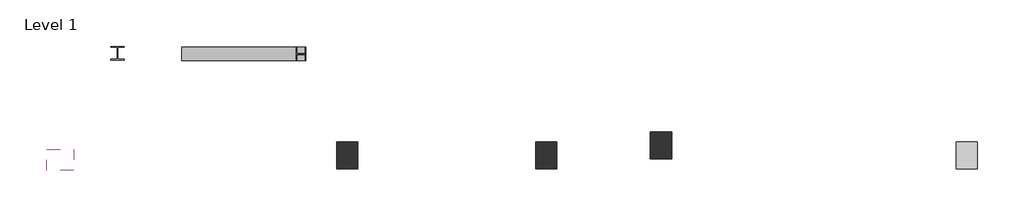
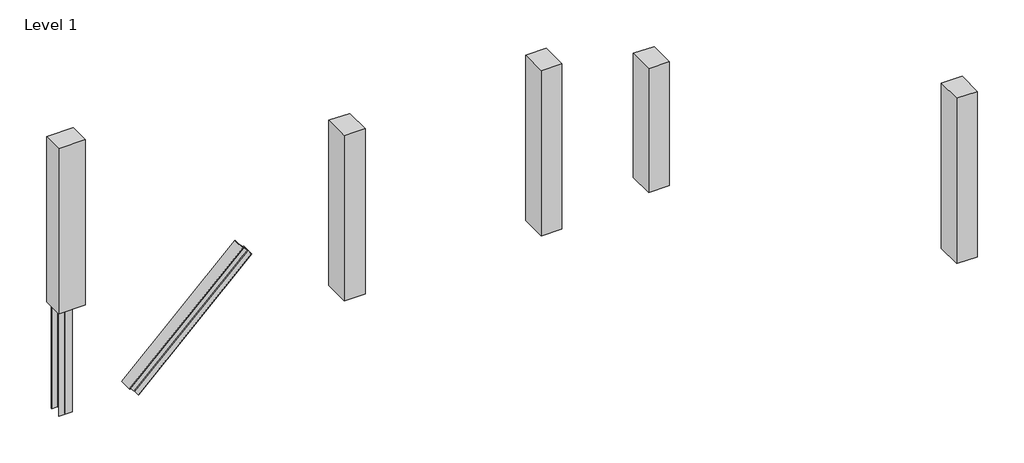
# One storey: 7 columns.
"""IFC4 building model written with IfcOpenShell, lengths in millimetres."""

import ifcopenshell
import ifcopenshell.guid

model = None  # the IFC model being written
_history = None  # IfcOwnerHistory: only IFC2X3 demands one
_inside = {}  # id of a spatial element -> (the spatial element, [elements in it])
_under = {}  # id of a project, library or spatial element -> (it, [spatial elements below it])
_declared = {}  # id of a project -> (the project, [libraries it declares])
_typed = {}  # id of a type object -> (the type object, [elements of that type])
_made_of = {}  # id of a material, layer set ... -> (it, [elements and type objects made of it])


def new_model(schema):
    """Start an empty IFC model of exactly this schema.

    Asked for "IFC4X3", IfcOpenShell would pick the latest addendum, in which some entities
    have other attributes; the version numbers below select the first issue.
    IFC2X3 requires an IfcOwnerHistory on every rooted entity: one is made here for all.
    """
    global model, _history
    if schema == "IFC4X3":
        model = ifcopenshell.file(schema_version=(4, 3, 0, 0))
    else:
        model = ifcopenshell.file(schema=schema)
    _inside.clear()
    _under.clear()
    _declared.clear()
    _typed.clear()
    _made_of.clear()
    _history = None
    if model.schema == "IFC2X3":
        org = make("IfcOrganization", Name="unknown")
        user = make(
            "IfcPersonAndOrganization",
            ThePerson=make("IfcPerson", FamilyName="unknown"),
            TheOrganization=org,
        )
        app = make(
            "IfcApplication",
            ApplicationDeveloper=org,
            Version="unknown",
            ApplicationFullName="unknown",
            ApplicationIdentifier="unknown",
        )
        _history = make(
            "IfcOwnerHistory",
            OwningUser=user,
            OwningApplication=app,
            ChangeAction="ADDED",
            CreationDate=0,
        )
    return model


def make(cls, **values):
    """One entity of the class cls with the attributes given. An attribute that is None is left unset."""
    return model.create_entity(
        cls, **{name: value for name, value in values.items() if value is not None}
    )


def rooted(cls, **values):
    """An entity with a GlobalId (a new one), such as an element, a storey or a relation."""
    return make(cls, GlobalId=ifcopenshell.guid.new(), OwnerHistory=_history, **values)


def si_unit(unit_type, name, prefix=None):
    """IfcSIUnit, for example si_unit("LENGTHUNIT", "METRE", prefix="MILLI")."""
    return make("IfcSIUnit", UnitType=unit_type, Prefix=prefix, Name=name)


def assignment(units):
    """IfcUnitAssignment: the units of a project."""
    return None if units is None else make("IfcUnitAssignment", Units=units)


def point(xyz):
    """IfcCartesianPoint."""
    return None if xyz is None else make("IfcCartesianPoint", Coordinates=xyz)


def direction(xyz):
    """IfcDirection."""
    return None if xyz is None else make("IfcDirection", DirectionRatios=xyz)


def frame(location, z_axis=None, x_axis=None):
    """IfcAxis2Placement3D, a coordinate frame: its origin and axes. An axis left out is left unset."""
    return make(
        "IfcAxis2Placement3D",
        Location=point(location),
        Axis=direction(z_axis),
        RefDirection=direction(x_axis),
    )


def frame_2d(location, x_axis=None):
    """IfcAxis2Placement2D, a coordinate frame in the plane: its origin and x axis."""
    return make(
        "IfcAxis2Placement2D", Location=point(location), RefDirection=direction(x_axis)
    )


def origin():
    """The frame at (0, 0, 0) with its axes left unset."""
    return frame((0.0, 0.0, 0.0))


def origin_with_axes():
    """The frame at (0, 0, 0) with the z axis (0, 0, 1) and the x axis (1, 0, 0) written out."""
    return frame((0.0, 0.0, 0.0), z_axis=(0.0, 0.0, 1.0), x_axis=(1.0, 0.0, 0.0))


def place(relative_to, where):
    """IfcLocalPlacement: puts the frame where relative to a parent placement (None: the world)."""
    return make(
        "IfcLocalPlacement", PlacementRelTo=relative_to, RelativePlacement=where
    )


def context(
    kind, dimensions, precision=None, world=None, true_north=None, identifier=None
):
    """IfcGeometricRepresentationContext, for example the 3D "Model" context."""
    return make(
        "IfcGeometricRepresentationContext",
        ContextIdentifier=identifier,
        ContextType=kind,
        CoordinateSpaceDimension=dimensions,
        Precision=precision,
        WorldCoordinateSystem=world,
        TrueNorth=true_north,
    )


def project(units=None, contexts=None):
    """IfcProject with its units and contexts."""
    return rooted(
        "IfcProject",
        Name="project",
        RepresentationContexts=contexts,
        UnitsInContext=assignment(units),
    )


def spatial(cls, under=None, at=None, **own):
    """A site, building, storey or space (cls), placed at a placement, below another one or the project."""
    s = rooted(cls, ObjectPlacement=at, **own)
    if under is not None:
        _under.setdefault(under.id(), (under, []))[1].append(s)
    return s


def polyline(points):
    """IfcPolyline through the points."""
    return make("IfcPolyline", Points=[point(p) for p in points])


def circle_curve(where, radius):
    """IfcCircle in the frame where."""
    return make("IfcCircle", Position=where, Radius=radius)


def trimmed(basis, trim1, trim2, sense, master):
    """IfcTrimmedCurve: the piece of a basis curve between two trims."""
    return make(
        "IfcTrimmedCurve",
        BasisCurve=basis,
        Trim1=trim1,
        Trim2=trim2,
        SenseAgreement=sense,
        MasterRepresentation=master,
    )


def segment(curve, same_sense, transition):
    """IfcCompositeCurveSegment."""
    return make(
        "IfcCompositeCurveSegment",
        Transition=transition,
        SameSense=same_sense,
        ParentCurve=curve,
    )


def composite_curve(segments, self_intersect=None):
    """IfcCompositeCurve: segments joined end to end."""
    return make("IfcCompositeCurve", Segments=segments, SelfIntersect=self_intersect)


def outline(outer, holes=None, kind="AREA"):
    """IfcArbitraryClosedProfileDef: a profile drawn as a closed curve; with holes, ...WithVoids."""
    if holes is None:
        return make("IfcArbitraryClosedProfileDef", ProfileType=kind, OuterCurve=outer)
    return make(
        "IfcArbitraryProfileDefWithVoids",
        ProfileType=kind,
        OuterCurve=outer,
        InnerCurves=holes,
    )


def extrude(swept, where, along, depth):
    """IfcExtrudedAreaSolid: the profile swept, set in the frame where, extruded along a direction by depth."""
    return make(
        "IfcExtrudedAreaSolid",
        SweptArea=swept,
        Position=where,
        ExtrudedDirection=direction(along),
        Depth=depth,
    )


def shape(context_of_items, identifier, shape_type, items):
    """IfcShapeRepresentation: the items that make up one representation, for example the "Body"."""
    return make(
        "IfcShapeRepresentation",
        ContextOfItems=context_of_items,
        RepresentationIdentifier=identifier,
        RepresentationType=shape_type,
        Items=items,
    )


def source(mapping_origin, context_of_items, identifier, shape_type, items):
    """IfcRepresentationMap: a shape defined once, which mapped items show again and again."""
    return make(
        "IfcRepresentationMap",
        MappingOrigin=mapping_origin,
        MappedRepresentation=shape(context_of_items, identifier, shape_type, items),
    )


def transform(
    local_origin,
    x_axis=None,
    y_axis=None,
    z_axis=None,
    scale=None,
    scale2=None,
    scale3=None,
    uniform=True,
):
    """IfcCartesianTransformationOperator3D, or its non-uniform kind. x_axis, y_axis, z_axis: its Axis1, 2, 3."""
    if uniform:
        return make(
            "IfcCartesianTransformationOperator3D",
            Axis1=direction(x_axis),
            Axis2=direction(y_axis),
            LocalOrigin=point(local_origin),
            Scale=scale,
            Axis3=direction(z_axis),
        )
    return make(
        "IfcCartesianTransformationOperator3DnonUniform",
        Axis1=direction(x_axis),
        Axis2=direction(y_axis),
        LocalOrigin=point(local_origin),
        Scale=scale,
        Axis3=direction(z_axis),
        Scale2=scale2,
        Scale3=scale3,
    )


def mapped(mapping_source, mapping_target):
    """IfcMappedItem: shows the shape of a source again, moved by a transform."""
    return make(
        "IfcMappedItem", MappingSource=mapping_source, MappingTarget=mapping_target
    )


def made_of(thing, what):
    """Note that an element or type object is made of a material, layer set ...; save() writes the relation."""
    if what is not None:
        _made_of.setdefault(what.id(), (what, []))[1].append(thing)
    return thing


def element(
    cls,
    number,
    at=None,
    inside=None,
    cuts=None,
    type_object=None,
    material=None,
    context=None,
    identifier="Body",
    shape_type=None,
    held_by="IfcProductDefinitionShape",
    body=None,
    shapes=None,
    **own,
):
    """One element of the class cls, such as IfcWall. Its Tag is "e" and its number.

    at: its placement. inside: the storey or other place that contains it. cuts: it is an
    opening in that element (IfcRelVoidsElement). A single representation is given by context,
    identifier, shape_type and body (its items); several are given by shapes. held_by: the class
    of the entity that holds the representations. save() writes the other relations.
    """
    e = rooted(cls, Tag="e%d" % number, ObjectPlacement=at, **own)
    if body is not None:
        shapes = [shape(context, identifier, shape_type, body)]
    if shapes is not None:
        e.Representation = make(held_by, Representations=shapes)
    if inside is not None:
        _inside.setdefault(inside.id(), (inside, []))[1].append(e)
    if cuts is not None:
        rooted(
            "IfcRelVoidsElement", RelatingBuildingElement=cuts, RelatedOpeningElement=e
        )
    if type_object is not None:
        _typed.setdefault(type_object.id(), (type_object, []))[1].append(e)
    return made_of(e, material)


def aggregate(whole, parts):
    """IfcRelAggregates: a whole, such as a stair, and the parts it consists of."""
    return rooted("IfcRelAggregates", RelatingObject=whole, RelatedObjects=parts)


def save(model, path):
    """Write the relations noted so far, then the file.

    IfcRelAggregates (storeys below a building ...), IfcRelContainedInSpatialStructure (elements
    in a storey), IfcRelDefinesByType, IfcRelAssociatesMaterial and IfcRelDeclares: one each for
    every whole, place, type object, material and project.
    """
    for whole, parts in _under.values():
        aggregate(whole, parts)
    for where, things in _inside.values():
        rooted(
            "IfcRelContainedInSpatialStructure",
            RelatedElements=things,
            RelatingStructure=where,
        )
    for kind, things in _typed.values():
        rooted("IfcRelDefinesByType", RelatedObjects=things, RelatingType=kind)
    for what, things in _made_of.values():
        rooted("IfcRelAssociatesMaterial", RelatedObjects=things, RelatingMaterial=what)
    for by, libraries in _declared.values():
        rooted("IfcRelDeclares", RelatingContext=by, RelatedDefinitions=libraries)
    model.write(path)


def m_rectangular_column_475_x_610mm_e62a7db6(model_context):
    return source(origin(), model_context, "Body", "SweptSolid", [
        extrude(outline(polyline([(305.0, 237.5), (305.0, -237.5), (-305.0, -237.5), (-305.0, 237.5), (305.0, 237.5)])), frame((0.0, 0.0, 2000.0), z_axis=(0.0, 0.0, 1.0), x_axis=(1.0, 0.0, 0.0)), (0.0, 0.0, 1.0), 4000.0),
    ])


def m_rectangular_column_475_x_610mm_b7c60445(model_context):
    return source(origin(), model_context, "Body", "SweptSolid", [
        extrude(outline(polyline([(305.0, 237.5), (305.0, -237.5), (-305.0, -237.5), (-305.0, 237.5), (305.0, 237.5)])), origin_with_axes(), (0.0, 0.0, 1.0), 4000.0),
    ])


def m_rectangular_column_475_x_610mm_f11b4c06(model_context):
    return source(origin(), model_context, "Body", "SweptSolid", [
        extrude(outline(polyline([(305.0, 237.5), (305.0, -237.5), (-305.0, -237.5), (-305.0, 237.5), (305.0, 237.5)])), origin_with_axes(), (0.0, 0.0, 1.0), 3000.0),
    ])


def m_rectangular_column_475_x_610mm_1e9c0db0(model_context):
    return source(origin(), model_context, "Body", "SweptSolid", [
        extrude(outline(polyline([(305.0, 237.5), (305.0, -237.5), (-305.0, -237.5), (-305.0, 237.5), (305.0, 237.5)])), frame((0.0, 0.0, -4000.0), z_axis=(0.0, 0.0, 1.0), x_axis=(1.0, 0.0, 0.0)), (0.0, 0.0, 1.0), 4000.0),
    ])


def uc_universal_columns_column_uc305x305x97_2af35403(model_context):
    return source(origin(), model_context, "Body", "SweptSolid", [
        extrude(outline(composite_curve([segment(polyline([(152.65, 153.95), (152.65, 138.55), (20.15, 138.55)]), True, "CONTINUOUS"), segment(trimmed(circle_curve(frame_2d((20.15, 123.35)), 15.2), [point((20.15, 138.55))], [point((4.95, 123.35))], True, "CARTESIAN"), True, "CONTINUOUS"), segment(polyline([(4.95, 123.35), (4.95, -123.35)]), True, "CONTINUOUS"), segment(trimmed(circle_curve(frame_2d((20.15, -123.35)), 15.2), [point((4.95, -123.35))], [point((20.15, -138.55))], True, "CARTESIAN"), True, "CONTINUOUS"), segment(polyline([(20.15, -138.55), (152.65, -138.55), (152.65, -153.95), (-152.65, -153.95), (-152.65, -138.55), (-20.15, -138.55)]), True, "CONTINUOUS"), segment(trimmed(circle_curve(frame_2d((-20.15, -123.35)), 15.2), [point((-20.15, -138.55))], [point((-4.95, -123.35))], True, "CARTESIAN"), True, "CONTINUOUS"), segment(polyline([(-4.95, -123.35), (-4.95, 123.35)]), True, "CONTINUOUS"), segment(trimmed(circle_curve(frame_2d((-20.15, 123.35)), 15.2), [point((-4.95, 123.35))], [point((-20.15, 138.55))], True, "CARTESIAN"), True, "CONTINUOUS"), segment(polyline([(-20.15, 138.55), (-152.65, 138.55), (-152.65, 153.95), (152.65, 153.95)]), True, "CONTINUOUS")], self_intersect=False)), frame((0.0, 0.0, -2500.0), z_axis=(0.0, 0.0, 1.0), x_axis=(1.0, 0.0, 0.0)), (0.0, 0.0, 1.0), 2500.0),
    ])


model = new_model("IFC4")

# Units and contexts
model_context = context("Model", 3, world=origin())
ifc_project = project(units=[si_unit("LENGTHUNIT", "METRE", prefix="MILLI")], contexts=[model_context])

# Site, building, storey
site = spatial("IfcSite", under=ifc_project)
building = spatial("IfcBuilding", under=site)
storey = spatial("IfcBuildingStorey", under=building, Name="Level 1", Elevation=0.0)

# Columns
placement = place(None, origin())
m_rectangular_column_475_x_610mm_shape = m_rectangular_column_475_x_610mm_e62a7db6(model_context)
element("IfcColumn", 1, ObjectType="M_Rectangular Column : 475 x 610mm", at=placement, inside=storey, context=model_context, shape_type="MappedRepresentation", body=[
    mapped(m_rectangular_column_475_x_610mm_shape, transform((-17655.4655243, 10194.8525449, 0.0), x_axis=(1.0, 0.0, 0.0), y_axis=(0.0, 1.0, 0.0), z_axis=(0.0, 0.0, 1.0))),
])
m_rectangular_column_475_x_610mm_2_shape = m_rectangular_column_475_x_610mm_b7c60445(model_context)
element("IfcColumn", 2, ObjectType="M_Rectangular Column : 475 x 610mm", at=placement, inside=storey, context=model_context, shape_type="MappedRepresentation", body=[
    mapped(m_rectangular_column_475_x_610mm_2_shape, transform((-11172.9984463, 10294.8525449, 0.0), x_axis=(0.0, 1.0, 0.0), y_axis=(-1.0, 0.0, 0.0), z_axis=(0.0, 0.0, 1.0))),
])
element("IfcColumn", 3, ObjectType="M_Rectangular Column : 475 x 610mm", at=placement, inside=storey, context=model_context, shape_type="MappedRepresentation", body=[
    mapped(m_rectangular_column_475_x_610mm_2_shape, transform((-6672.9984463, 10294.8525449, 0.0), x_axis=(0.0, 1.0, 0.0), y_axis=(-1.0, 0.0, 0.0), z_axis=(0.0, 0.0, 1.0))),
])
m_rectangular_column_475_x_610mm_3_shape = m_rectangular_column_475_x_610mm_f11b4c06(model_context)
element("IfcColumn", 4, ObjectType="M_Rectangular Column : 475 x 610mm", at=placement, inside=storey, context=model_context, shape_type="MappedRepresentation", body=[
    mapped(m_rectangular_column_475_x_610mm_3_shape, transform((-4082.8922313, 10521.457476, 0.0), x_axis=(0.0, 1.0, 0.0), y_axis=(-1.0, 0.0, 0.0), z_axis=(0.0, 0.0, 1.0))),
])
m_rectangular_column_475_x_610mm_4_shape = m_rectangular_column_475_x_610mm_1e9c0db0(model_context)
element("IfcColumn", 5, ObjectType="M_Rectangular Column : 475 x 610mm", at=placement, inside=storey, context=model_context, shape_type="MappedRepresentation", body=[
    mapped(m_rectangular_column_475_x_610mm_4_shape, transform((2827.0015537, 10294.8525449, 0.0), x_axis=(0.0, 1.0, 0.0), y_axis=(-1.0, 0.0, 0.0), z_axis=(0.0, 0.0, 1.0))),
])
element("IfcColumn", 6, ObjectType="UC-Universal Columns-Column : UC305x305x97", at=placement, inside=storey, context=model_context, shape_type="SweptSolid", body=[
    extrude(outline(composite_curve([segment(polyline([(305.3, 0.0), (305.3, -15.4), (172.8, -15.4)]), True, "CONTINUOUS"), segment(trimmed(circle_curve(frame_2d((172.8, -30.6)), 15.2), [point((172.8, -15.4))], [point((157.6, -30.6))], True, "CARTESIAN"), True, "CONTINUOUS"), segment(polyline([(157.6, -30.6), (157.6, -277.3000001)]), True, "CONTINUOUS"), segment(trimmed(circle_curve(frame_2d((172.8, -277.3000001)), 15.2), [point((157.6, -277.3000001))], [point((172.8, -292.5))], True, "CARTESIAN"), True, "CONTINUOUS"), segment(polyline([(172.8, -292.5), (305.3, -292.5), (305.3, -307.9), (0.0, -307.9), (0.0, -292.5), (132.5, -292.5)]), True, "CONTINUOUS"), segment(trimmed(circle_curve(frame_2d((132.5, -277.3000001)), 15.2), [point((132.5, -292.5))], [point((147.7, -277.3000001))], True, "CARTESIAN"), True, "CONTINUOUS"), segment(polyline([(147.7, -277.3000001), (147.7, -30.6)]), True, "CONTINUOUS"), segment(trimmed(circle_curve(frame_2d((132.5, -30.6)), 15.2), [point((147.7, -30.6))], [point((132.5, -15.4))], True, "CARTESIAN"), True, "CONTINUOUS"), segment(polyline([(132.5, -15.4), (0.0, -15.4), (0.0, 0.0), (305.3, 0.0)]), True, "CONTINUOUS")], self_intersect=False)), frame((-14909.4462921, 12442.2025449, -2389.2258433), z_axis=(0.7195463248327014, 0.0, 0.6944444444444441), x_axis=(0.0, 1.0, 0.0)), (0.0, 0.0, 1.0), 3600.0),
])
uc_universal_columns_column_uc305x305x97_shape = uc_universal_columns_column_uc305x305x97_2af35403(model_context)
element("IfcColumn", 7, ObjectType="UC-Universal Columns-Column : UC305x305x97", at=placement, inside=storey, context=model_context, shape_type="MappedRepresentation", body=[
    mapped(uc_universal_columns_column_uc305x305x97_shape, transform((-16355.4655243, 12612.2564061, 0.0), x_axis=(1.0, 0.0, 0.0), y_axis=(0.0, 1.0, 0.0), z_axis=(0.0, 0.0, 1.0))),
])

save(model, "model.ifc")

# Revit data of these elements
# Project information
#   Project Issue Date = "Issue Date"
#   Project Status = "Project Status"
#   Client Name = "Owner"
#   Project Address = "Enter address here"
#   Project Name = "Project Name"
#   Project Number = "0001"
# Type "M_Rectangular Column : 475 x 610mm"
#   Depth = 475 mm
#   Offset Base = 0 mm
#   Offset Top = 0 mm
#   Width = 610 mm
#   Material = none
# Type "UC-Universal Columns-Column : UC305x305x97"
#   Section Name Key = "UC305x305x97"
#   Width = 30.53 cm
#   Web Thickness = 0.99 cm
#   Web Fillet = 1.52 cm
#   Warping Constant = 1560000.0 cm⁶
#   Torsional Moment of Inertia = 91.20 cm⁴
#   Section Area = 123.0 cm²
#   Plastic Modulus weak axis = 726.0 cm³
#   Plastic Modulus strong axis = 1592.0 cm³
#   Nominal Weight = 96.8996 kgf/m
#   Moment of Inertia weak axis = 7308.00 cm⁴
#   Moment of Inertia strong axis = 22249.00 cm⁴
#   Height = 30.79 cm
#   Flange Thickness = 1.54 cm
#   Elastic Modulus weak axis = 479.0 cm³
#   Elastic Modulus strong axis = 1445.0 cm³
#   Centroid Vertical = 15.395 cm
#   Centroid Horizontal = 15.265 cm
#   Bolt Spacing = 14.0 cm
#   Structural Material [instance default] = Metal - Steel 43-275
#   Type Comments = ""
#   Assembly Code = ""
# Element 1 (IfcColumn, "M_Rectangular Column : 475 x 610mm")
#   SpeckleObjectTestNumber = 1
#   Phase Created = New Construction
# Element 2 (IfcColumn, "M_Rectangular Column : 475 x 610mm")
#   SpeckleObjectTestNumber = 4
#   Phase Created = New Construction
# Element 3 (IfcColumn, "M_Rectangular Column : 475 x 610mm")
#   SpeckleObjectTestNumber = 6
#   Phase Created = New Construction
# Element 4 (IfcColumn, "M_Rectangular Column : 475 x 610mm")
#   SpeckleObjectTestNumber = 7
#   Phase Created = New Construction
# Element 5 (IfcColumn, "M_Rectangular Column : 475 x 610mm")
#   SpeckleObjectTestNumber = 9
#   Phase Created = New Construction
# Element 6 (IfcColumn, "UC-Universal Columns-Column : UC305x305x97")
#   SpeckleObjectTestNumber = 3
#   Structural Material = Metal - Steel 43-275
#   Phase Created = New Construction
#   Materials on its faces: "Metal - Steel 43-275"
# Element 7 (IfcColumn, "UC-Universal Columns-Column : UC305x305x97")
#   SpeckleObjectTestNumber = 2
#   Structural Material = Metal - Steel 43-275
#   Phase Created = New Construction
#   Materials on its faces: "Metal - Steel 43-275"
# Materials
#   "Metal - Steel 43-275": class "Metal", colour RGB 247 247 247, transparency 0, Cost = 0
